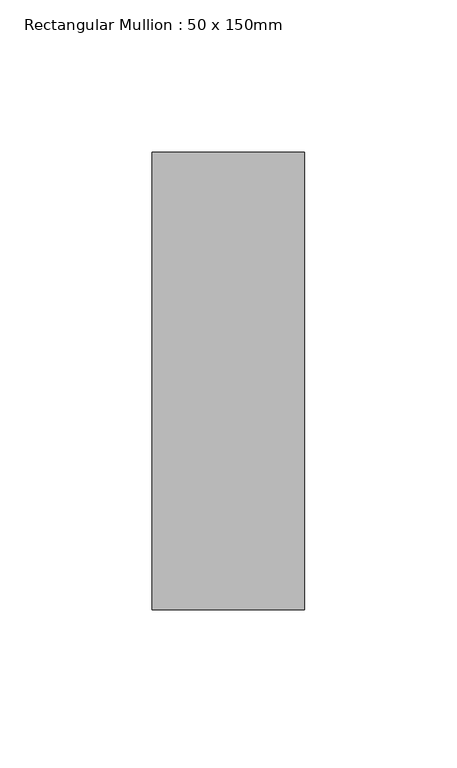
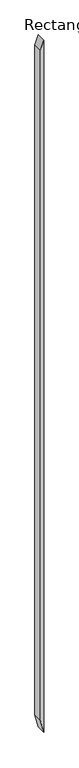
"""IFC4 building model written with IfcOpenShell, lengths in millimetres: member geometry, Rectangular Mullion : 50 x 150mm."""

from ifc_helpers import new_model, si_unit, frame, origin, place, context, project, spatial, polyline, outline, extrude, source, transform, mapped, element, save


def rectangular_mullion_50_x_150mm_26c19414(model_context):
    return source(origin(), model_context, "Body", "SweptSolid", [
        extrude(outline(polyline([(0.0, 0.0), (-156.788361, -50.0), (-11226.8029982, -50.0), (-11440.3058664, 0.0), (0.0, 0.0)])), frame((0.0, -75.0, 0.0), z_axis=(0.0, 1.0, 0.0), x_axis=(0.0, 0.0, 1.0)), (0.0, 0.0, 1.0), 150.0),
    ])


if __name__ == "__main__":
    model = new_model("IFC4")
    model_context = context("Model", 3, world=origin())
    ifc_project = project(units=[si_unit("LENGTHUNIT", "METRE", prefix="MILLI")], contexts=[model_context])
    site = spatial("IfcSite", under=ifc_project)
    building = spatial("IfcBuilding", under=site)
    placement = place(None, origin())
    rectangular_mullion_50_x_150mm_shape = rectangular_mullion_50_x_150mm_26c19414(model_context)
    element("IfcMember", 1, ObjectType="Rectangular Mullion : 50 x 150mm", at=placement, inside=building, context=model_context, shape_type="MappedRepresentation", body=[
        mapped(rectangular_mullion_50_x_150mm_shape, transform((0.0, 0.0, 0.0), x_axis=(1.0, 0.0, 0.0), y_axis=(0.0, 1.0, 0.0), z_axis=(0.0, 0.0, 1.0))),
    ])
    save(model, "model.ifc")

# Revit data of these elements
# Type "Rectangular Mullion : 50 x 150mm"
#   built-in parameter 1007304 = 0.492126 (stored number, unit not read)
#   built-in parameter 1007301 = 0.082021 (stored number, unit not read)
#   built-in parameter 1007300 = 0.082021 (stored number, unit not read)
# Element 1 (IfcMember, "Rectangular Mullion : 50 x 150mm")
#   Materials on its faces: "Metal - Aluminium"
# Materials
#   "Metal - Aluminium": class "Metal", colour RGB 247 247 247, transparency 0
